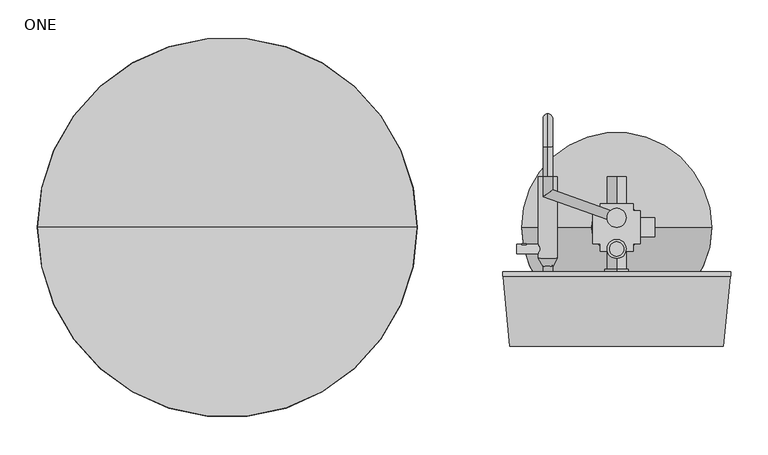
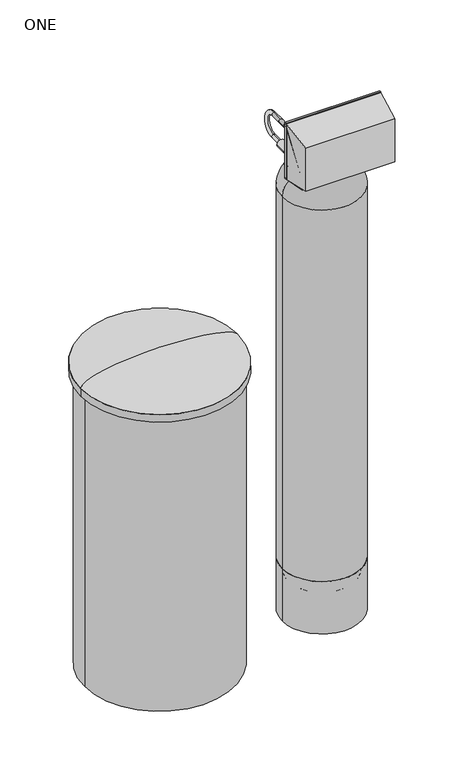
"""IFC4 building model written with IfcOpenShell, lengths in millimetres: proxy geometry, Water_Softener-Single-Robert_B_Hill-Fiberglass : ONE."""

from ifc_helpers import new_model, si_unit, point, frame, frame_2d, origin, origin_with_axes, place, context, project, spatial, polyline, circle_curve, ellipse_curve, trimmed, segment, composite_curve, outline, extrude, faceted_brep, source, transform, mapped, element, save
from ifc_brep_helpers import plane_surface, cylinder_surface, revolved_surface, advanced_brep


def one_3beddf22(model_context):
    return source(origin(), model_context, "Body", "SolidModel", [
        extrude(outline(composite_curve([segment(trimmed(circle_curve(frame_2d((203.2, -28.956)), 9.525), [point((212.725, -28.956))], [point((193.675, -28.956))], False, "CARTESIAN"), True, "CONTINUOUS"), segment(trimmed(circle_curve(frame_2d((203.2, -28.956)), 9.525), [point((193.675, -28.956))], [point((212.725, -28.956))], False, "CARTESIAN"), True, "CONTINUOUS")], self_intersect=False)), frame((0.0, 0.0, 1608.455), z_axis=(0.0, 0.0, 1.0), x_axis=(1.0, 0.0, 0.0)), (0.0, 0.0, 1.0), 19.05),
        extrude(outline(composite_curve([segment(trimmed(circle_curve(frame_2d((0.0, 1581.15)), 9.525), [point((0.0, 1571.625))], [point((0.0, 1590.675))], False, "CARTESIAN"), True, "CONTINUOUS"), segment(trimmed(circle_curve(frame_2d((0.0, 1581.15)), 9.525), [point((0.0, 1590.675))], [point((0.0, 1571.625))], False, "CARTESIAN"), True, "CONTINUOUS")], self_intersect=False)), frame((231.775, 0.0, 0.0), z_axis=(1.0, 0.0, 0.0), x_axis=(0.0, 1.0, 0.0)), (0.0, 0.0, 1.0), 19.05),
        advanced_brep(
        [(203.2, -55.9279754, 1581.15), (203.2, -55.9279754, 1555.75), (203.2, -55.9279754, 1552.575), (203.2, -55.9279754, 1584.325), (203.2, 67.8970246, 1581.15), (203.2, 67.8970246, 1555.75), (203.2, 67.8970246, 1568.45), (203.2, -59.1029754, 1584.325), (203.2, -59.1029754, 1552.575), (203.2, -59.1029754, 1568.45)],
        [
            (0, 1, circle_curve(frame((203.2, -55.9279754, 1568.45), z_axis=(0.0, -1.0, 0.0), x_axis=(0.0, 0.0, -1.0)), 12.7)),
            (1, 2),
            (2, 3, circle_curve(frame((203.2, -55.9279754, 1568.45), z_axis=(0.0, 1.0, 0.0), x_axis=(0.0, 0.0, -1.0)), 15.875)),
            (3, 0),
            (1, 0, circle_curve(frame((203.2, -55.9279754, 1568.45), z_axis=(0.0, -1.0, 0.0), x_axis=(0.0, 0.0, -1.0)), 12.7)),
            (3, 2, circle_curve(frame((203.2, -55.9279754, 1568.45), z_axis=(0.0, 1.0, 0.0), x_axis=(0.0, 0.0, -1.0)), 15.875)),
            (4, 5, circle_curve(frame((203.2, 67.8970246, 1568.45), z_axis=(0.0, -1.0, 0.0), x_axis=(0.0, 0.0, -1.0)), 12.7)),
            (5, 1),
            (0, 4),
            (5, 4, circle_curve(frame((203.2, 67.8970246, 1568.45), z_axis=(0.0, -1.0, 0.0), x_axis=(0.0, 0.0, -1.0)), 12.7)),
            (6, 5),
            (4, 6),
            (7, 8, circle_curve(frame((203.2, -59.1029754, 1568.45), z_axis=(0.0, -1.0, 0.0), x_axis=(0.0, 0.0, -1.0)), 15.875)),
            (8, 9),
            (9, 7),
            (8, 7, circle_curve(frame((203.2, -59.1029754, 1568.45), z_axis=(0.0, -1.0, 0.0), x_axis=(0.0, 0.0, -1.0)), 15.875)),
            (2, 8),
            (7, 3),
        ],
        [
            plane_surface(frame((203.2, -55.9279754, 1568.45), z_axis=(0.0, 1.0, 0.0), x_axis=(0.0, 0.0, -1.0))),
            cylinder_surface(frame((203.2, -59.1029754, 1568.45), z_axis=(0.0, 1.0, 0.0), x_axis=(0.0, 0.0, -1.0)), 12.7),
            plane_surface(frame((203.2, 67.8970246, 1568.45), z_axis=(0.0, 1.0, 0.0), x_axis=(0.0, 0.0, -1.0))),
            plane_surface(frame((203.2, -59.1029754, 1568.45), z_axis=(0.0, -1.0, 0.0), x_axis=(0.0, 0.0, -1.0))),
            cylinder_surface(frame((203.2, -59.1029754, 1568.45), z_axis=(0.0, 1.0, 0.0), x_axis=(0.0, 0.0, -1.0)), 15.875),
        ],
        [
            (0, [[1, 2, 3, 4]]),
            (0, [[5, -4, 6, -2]]),
            (1, [[7, 8, -1, 9]]),
            (1, [[10, -9, -5, -8]]),
            (2, [[11, -7, 12]]),
            (2, [[-12, -10, -11]]),
            (3, [[13, 14, 15]]),
            (3, [[16, -15, -14]]),
            (4, [[-3, 17, -13, 18]]),
            (4, [[-6, -18, -16, -17]]),
        ],
    ),
        extrude(outline(polyline([(1738.3125, 355.6), (1738.3125, 50.8), (1552.575, 50.8), (1552.575, 355.6), (1738.3125, 355.6)]), holes=[polyline([(1558.925, 349.25), (1558.925, 57.15), (1731.9625, 57.15), (1731.9625, 349.25), (1558.925, 349.25)])]), frame((0.0, -65.4529754, 0.0), z_axis=(0.0, 1.0, 0.0), x_axis=(0.0, 0.0, 1.0)), (0.0, 0.0, 1.0), 6.35),
        faceted_brep([(346.075, -140.1006819, 1552.575), (346.075, -140.1006819, 1589.4295859), (60.325, -140.1006819, 1589.4295859), (60.325, -140.1006819, 1552.575), (355.6, -59.1029754, 1547.8125), (50.8, -59.1029754, 1547.8125), (50.8, -59.1029754, 1738.3125), (355.6, -59.1029754, 1738.3125)], [[[0, 1, 2, 3]], [[4, 5, 6, 7]], [[4, 7, 1, 0]], [[7, 6, 2, 1]], [[6, 5, 3, 2]], [[5, 4, 0, 3]]]),
        extrude(outline(composite_curve([segment(trimmed(circle_curve(frame_2d((203.2, 0.0)), 31.75), [point((171.45, 0.0))], [point((234.95, 0.0))], False, "CARTESIAN"), True, "CONTINUOUS"), segment(trimmed(circle_curve(frame_2d((203.2, 0.0)), 31.75), [point((234.95, 0.0))], [point((171.45, 0.0))], False, "CARTESIAN"), True, "CONTINUOUS")], self_intersect=False)), frame((0.0, 0.0, 1536.7), z_axis=(0.0, 0.0, 1.0), x_axis=(1.0, 0.0, 0.0)), (0.0, 0.0, 1.0), 24.1545859),
        faceted_brep([(60.325, -159.1154754, 1706.9045859), (60.325, -159.1154754, 1560.8545859), (346.075, -159.1154754, 1560.8545859), (346.075, -159.1154754, 1706.9045859), (50.8, -59.1029754, 1738.3125), (355.6, -59.1029754, 1738.3125), (355.6, -59.1029754, 1547.8125), (50.8, -59.1029754, 1547.8125)], [[[0, 1, 2, 3]], [[4, 5, 6, 7]], [[4, 7, 1, 0]], [[7, 6, 2, 1]], [[6, 5, 3, 2]], [[5, 4, 0, 3]]]),
        extrude(outline(composite_curve([segment(trimmed(circle_curve(frame_2d((1568.45, 111.125)), 6.35), [point((1568.45, 117.475))], [point((1568.45, 104.775))], False, "CARTESIAN"), True, "CONTINUOUS"), segment(trimmed(circle_curve(frame_2d((1568.45, 111.125)), 6.35), [point((1568.45, 104.775))], [point((1568.45, 117.475))], False, "CARTESIAN"), True, "CONTINUOUS")], self_intersect=False)), frame((0.0, -59.1029754, 0.0), z_axis=(0.0, 1.0, 0.0), x_axis=(0.0, 0.0, 1.0)), (0.0, 0.0, 1.0), 17.4625),
        extrude(outline(composite_curve([segment(trimmed(circle_curve(frame_2d((-28.9404754, 1568.45)), 6.35), [point((-35.2904754, 1568.45))], [point((-22.5904754, 1568.45))], False, "CARTESIAN"), True, "CONTINUOUS"), segment(trimmed(circle_curve(frame_2d((-28.9404754, 1568.45)), 6.35), [point((-22.5904754, 1568.45))], [point((-35.2904754, 1568.45))], False, "CARTESIAN"), True, "CONTINUOUS")], self_intersect=False)), frame((69.85, 0.0, 0.0), z_axis=(1.0, 0.0, 0.0), x_axis=(0.0, 1.0, 0.0)), (0.0, 0.0, 1.0), 41.275),
        extrude(outline(composite_curve([segment(trimmed(circle_curve(frame_2d((1568.45, 111.125)), 12.7), [point((1568.45, 98.425))], [point((1568.45, 123.825))], False, "CARTESIAN"), True, "CONTINUOUS"), segment(trimmed(circle_curve(frame_2d((1568.45, 111.125)), 12.7), [point((1568.45, 123.825))], [point((1568.45, 98.425))], False, "CARTESIAN"), True, "CONTINUOUS")], self_intersect=False)), frame((0.0, -41.6404754, 0.0), z_axis=(0.0, 1.0, 0.0), x_axis=(0.0, 0.0, 1.0)), (0.0, 0.0, 1.0), 109.5375),
        advanced_brep(
        [(98.425, -41.6404754, 1568.45), (123.825, -41.6404754, 1568.45), (104.775, -52.7529754, 1568.45), (117.475, -52.7529754, 1568.45)],
        [
            (0, 1, circle_curve(frame((111.125, -41.6404754, 1568.45), z_axis=(0.0, 1.0, 0.0), x_axis=(-1.0, 0.0, 0.0)), 12.7)),
            (1, 0, circle_curve(frame((111.125, -41.6404754, 1568.45), z_axis=(0.0, 1.0, 0.0), x_axis=(1.0, 0.0, 0.0)), 12.7)),
            (2, 3, circle_curve(frame((111.125, -52.7529754, 1568.45), z_axis=(0.0, -1.0, 0.0), x_axis=(1.0, 0.0, 0.0)), 6.35)),
            (3, 2, circle_curve(frame((111.125, -52.7529754, 1568.45), z_axis=(0.0, -1.0, 0.0), x_axis=(-1.0, 0.0, 0.0)), 6.35)),
            (2, 0),
            (1, 3),
        ],
        [
            plane_surface(frame((111.125, -41.6404754, 1568.45), z_axis=(0.0, 1.0, 0.0), x_axis=(0.0, 0.0, -1.0))),
            plane_surface(frame((111.125, -52.7529754, 1568.45), z_axis=(0.0, -1.0, 0.0), x_axis=(0.0, 0.0, -1.0))),
            revolved_surface(polyline([(104.77499999999999, -52.7529754, 1568.45), (98.425, -41.6404754, 1568.45)]), (111.125, -63.8654754, 1568.45), (0.0, 1.0, 0.0)),
            revolved_surface(polyline([(117.47500000000001, -52.7529754, 1568.45), (123.825, -41.6404754, 1568.45)]), (111.125, -63.8654754, 1568.45), (0.0, 1.0, 0.0)),
        ],
        [
            (0, [[1, 2]]),
            (1, [[3, 4]]),
            (2, [[-3, 5, -2, 6]]),
            (3, [[-4, -6, -1, -5]]),
        ],
    ),
        extrude(outline(composite_curve([segment(trimmed(circle_curve(frame_2d((203.2, 12.7)), 12.7), [point((190.5, 12.7))], [point((215.9, 12.7))], False, "CARTESIAN"), True, "CONTINUOUS"), segment(trimmed(circle_curve(frame_2d((203.2, 12.7)), 12.7), [point((215.9, 12.7))], [point((190.5, 12.7))], False, "CARTESIAN"), True, "CONTINUOUS")], self_intersect=False)), frame((0.0, 0.0, 1600.2), z_axis=(0.0, 0.0, 1.0), x_axis=(1.0, 0.0, 0.0)), (0.0, 0.0, 1.0), 60.325),
        advanced_brep(
        [(104.775, 67.8970246, 1644.65), (117.475, 67.8970246, 1644.65), (104.775, 41.2010874, 1644.65), (117.475, 50.1429618, 1644.65), (201.0591918, 6.7217527, 1644.65), (205.3408082, 18.6782473, 1644.65)],
        [
            (0, 1, circle_curve(frame((111.125, 67.8970246, 1644.65), z_axis=(0.0, 1.0, 0.0), x_axis=(1.0, 0.0, 0.0)), 6.35)),
            (1, 0, circle_curve(frame((111.125, 67.8970246, 1644.65), z_axis=(0.0, 1.0, 0.0), x_axis=(1.0, 0.0, 0.0)), 6.35)),
            (0, 2),
            (2, 3, ellipse_curve(frame((111.125, 45.6720246, 1644.65), z_axis=(-0.5757016803912287, 0.8176598163018136, 0.0), x_axis=(0.8176598163018136, 0.5757016803912287, 0.0)), 7.7660659, 6.35)),
            (3, 1),
            (3, 2, ellipse_curve(frame((111.125, 45.6720246, 1644.65), z_axis=(-0.5757016803912287, 0.8176598163018136, 0.0), x_axis=(0.8176598163018136, 0.5757016803912287, 0.0)), 7.7660659, 6.35)),
            (4, 5, circle_curve(frame((203.2, 12.7, 1644.65), z_axis=(0.941456260466675, -0.3371351503894311, 0.0), x_axis=(0.3371351503894311, 0.941456260466675, 0.0)), 6.35)),
            (5, 4, circle_curve(frame((203.2, 12.7, 1644.65), z_axis=(0.941456260466675, -0.3371351503894311, 0.0), x_axis=(0.3371351503894311, 0.941456260466675, 0.0)), 6.35)),
            (2, 4),
            (5, 3),
        ],
        [
            plane_surface(frame((111.125, 67.8970246, 1536.7), z_axis=(0.0, 1.0, 0.0), x_axis=(0.0, 0.0, 1.0))),
            cylinder_surface(frame((111.125, 67.8970246, 1644.65), z_axis=(0.0, 1.0, 0.0), x_axis=(1.0, 0.0, 0.0)), 6.35),
            plane_surface(frame((203.2, 12.7, 1536.7), z_axis=(0.941456260466675, -0.3371351503894311, 0.0), x_axis=(0.0, 0.0, 1.0))),
            cylinder_surface(frame((111.125, 45.6720246, 1644.65), z_axis=(-0.941456260466675, 0.3371351503894311, 0.0), x_axis=(0.3371351503894311, 0.941456260466675, 0.0)), 6.35),
        ],
        [
            (0, [[1, 2]]),
            (1, [[-1, 3, 4, 5]]),
            (1, [[-2, -5, 6, -3]]),
            (2, [[7, 8]]),
            (3, [[-4, 9, -8, 10]]),
            (3, [[-6, -10, -7, -9]]),
        ],
    ),
        advanced_brep(
        [(111.125, -59.1029754, 1562.1), (111.125, -59.1029754, 1574.8), (111.125, 107.5845246, 1562.1), (111.125, 107.5845246, 1574.8), (111.125, 107.5845246, 1638.3), (111.125, 107.5845246, 1651.0), (111.125, 67.8970246, 1651.0), (111.125, 67.8970246, 1638.3)],
        [
            (0, 1, circle_curve(frame((111.125, -59.1029754, 1568.45), z_axis=(0.0, -1.0, 0.0), x_axis=(0.0, 0.0, 1.0)), 6.35)),
            (1, 0, circle_curve(frame((111.125, -59.1029754, 1568.45), z_axis=(0.0, -1.0, 0.0), x_axis=(0.0, 0.0, 1.0)), 6.35)),
            (0, 2),
            (2, 3, circle_curve(frame((111.125, 107.5845246, 1568.45), z_axis=(0.0, -1.0, 0.0), x_axis=(0.0, 0.0, 1.0)), 6.35)),
            (3, 1),
            (3, 2, circle_curve(frame((111.125, 107.5845246, 1568.45), z_axis=(0.0, -1.0, 0.0), x_axis=(0.0, 0.0, 1.0)), 6.35)),
            (4, 3, circle_curve(frame((111.125, 107.5845246, 1606.55), z_axis=(-1.0, 0.0, 0.0), x_axis=(0.0, 0.0, -1.0)), 31.75)),
            (2, 5, circle_curve(frame((111.125, 107.5845246, 1606.55), z_axis=(1.0, 0.0, 0.0), x_axis=(0.0, 0.0, -1.0)), 44.45)),
            (5, 4, circle_curve(frame((111.125, 107.5845246, 1644.65), z_axis=(0.0, 1.0, 0.0), x_axis=(0.0, 0.0, -1.0)), 6.35)),
            (4, 5, circle_curve(frame((111.125, 107.5845246, 1644.65), z_axis=(0.0, 1.0, 0.0), x_axis=(0.0, 0.0, -1.0)), 6.35)),
            (6, 7, circle_curve(frame((111.125, 67.8970246, 1644.65), z_axis=(0.0, -1.0, 0.0), x_axis=(0.0, 0.0, -1.0)), 6.35)),
            (7, 6, circle_curve(frame((111.125, 67.8970246, 1644.65), z_axis=(0.0, -1.0, 0.0), x_axis=(0.0, 0.0, -1.0)), 6.35)),
            (5, 6),
            (7, 4),
        ],
        [
            plane_surface(frame((203.2, -59.1029754, 1568.45), z_axis=(0.0, -1.0, 0.0), x_axis=(1.0, 0.0, 0.0))),
            cylinder_surface(frame((111.125, -59.1029754, 1568.45), z_axis=(0.0, -1.0, 0.0), x_axis=(0.0, 0.0, 1.0)), 6.35),
            revolved_surface(trimmed(ellipse_curve(frame((111.125, 107.5845246, 1568.45), z_axis=(0.0, -1.0, 0.0), x_axis=(0.0, 0.0, 1.0)), 6.35, 6.35), [point((111.125, 107.5845246, 1562.1))], [point((111.125, 107.5845246, 1574.8))], True, "CARTESIAN"), (203.2, 107.5845246, 1606.55), (1.0, 0.0, 0.0)),
            revolved_surface(trimmed(ellipse_curve(frame((111.125, 107.5845246, 1568.45), z_axis=(0.0, -1.0, 0.0), x_axis=(0.0, 0.0, 1.0)), 6.35, 6.35), [point((111.125, 107.5845246, 1574.8))], [point((111.125, 107.5845246, 1562.1))], True, "CARTESIAN"), (203.2, 107.5845246, 1606.55), (1.0, 0.0, 0.0)),
            plane_surface(frame((203.2, 67.8970246, 1644.65), z_axis=(0.0, -1.0, 0.0), x_axis=(1.0, 0.0, 0.0))),
            cylinder_surface(frame((111.125, 107.5845246, 1644.65), z_axis=(0.0, 1.0, 0.0), x_axis=(0.0, 0.0, -1.0)), 6.35),
        ],
        [
            (0, [[1, 2]]),
            (1, [[-1, 3, 4, 5]]),
            (1, [[-2, -5, 6, -3]]),
            (2, [[7, -4, 8, 9]]),
            (3, [[-8, -6, -7, 10]]),
            (4, [[11, 12]]),
            (5, [[-9, 13, -12, 14]]),
            (5, [[-10, -14, -11, -13]]),
        ],
    ),
        extrude(outline(polyline([(180.975, 22.225), (180.975, 31.75), (225.425, 31.75), (225.425, 22.225), (234.95, 22.225), (234.95, -22.225), (225.425, -22.225), (225.425, -31.75), (180.975, -31.75), (180.975, -22.225), (171.45, -22.225), (171.45, 22.225), (180.975, 22.225)])), frame((0.0, 0.0, 1552.575), z_axis=(0.0, 0.0, 1.0), x_axis=(1.0, 0.0, 0.0)), (0.0, 0.0, 1.0), 47.625),
        extrude(outline(composite_curve([segment(trimmed(circle_curve(frame_2d((203.2, -28.9404754)), 12.7), [point((190.5, -28.9404754))], [point((215.9, -28.9404754))], False, "CARTESIAN"), True, "CONTINUOUS"), segment(trimmed(circle_curve(frame_2d((203.2, -28.9404754)), 12.7), [point((215.9, -28.9404754))], [point((190.5, -28.9404754))], False, "CARTESIAN"), True, "CONTINUOUS")], self_intersect=False)), frame((0.0, 0.0, 1568.45), z_axis=(0.0, 0.0, 1.0), x_axis=(1.0, 0.0, 0.0)), (0.0, 0.0, 1.0), 59.0795859),
        extrude(outline(composite_curve([segment(trimmed(circle_curve(frame_2d((0.0, 1581.15)), 12.7), [point((-12.7, 1581.15))], [point((12.7, 1581.15))], False, "CARTESIAN"), True, "CONTINUOUS"), segment(trimmed(circle_curve(frame_2d((0.0, 1581.15)), 12.7), [point((12.7, 1581.15))], [point((-12.7, 1581.15))], False, "CARTESIAN"), True, "CONTINUOUS")], self_intersect=False)), frame((234.95, 0.0, 0.0), z_axis=(1.0, 0.0, 0.0), x_axis=(0.0, 1.0, 0.0)), (0.0, 0.0, 1.0), 19.05),
        advanced_brep(
        [(76.2, 0.0, 0.0), (330.2, 0.0, 0.0), (311.15, 0.0, 0.0), (95.25, 0.0, 0.0), (76.2, 0.0, 177.8), (330.2, 0.0, 177.8), (95.25, 0.0, 177.8), (311.15, 0.0, 177.8)],
        [
            (0, 1, circle_curve(frame((203.2, 0.0, 0.0), z_axis=(0.0, 0.0, -1.0), x_axis=(1.0, 0.0, 0.0)), 127.0)),
            (1, 2),
            (2, 3, circle_curve(frame((203.2, 0.0, 0.0), z_axis=(0.0, 0.0, 1.0), x_axis=(1.0, 0.0, 0.0)), 107.95)),
            (3, 0),
            (1, 0, circle_curve(frame((203.2, 0.0, 0.0), z_axis=(0.0, 0.0, -1.0), x_axis=(1.0, 0.0, 0.0)), 127.0)),
            (3, 2, circle_curve(frame((203.2, 0.0, 0.0), z_axis=(0.0, 0.0, 1.0), x_axis=(1.0, 0.0, 0.0)), 107.95)),
            (4, 5, circle_curve(frame((203.2, 0.0, 177.8), z_axis=(0.0, 0.0, -1.0), x_axis=(1.0, 0.0, 0.0)), 127.0)),
            (5, 1),
            (0, 4),
            (5, 4, circle_curve(frame((203.2, 0.0, 177.8), z_axis=(0.0, 0.0, -1.0), x_axis=(1.0, 0.0, 0.0)), 127.0)),
            (6, 7, circle_curve(frame((203.2, 0.0, 177.8), z_axis=(0.0, 0.0, -1.0), x_axis=(1.0, 0.0, 0.0)), 107.95)),
            (7, 5),
            (4, 6),
            (7, 6, circle_curve(frame((203.2, 0.0, 177.8), z_axis=(0.0, 0.0, -1.0), x_axis=(1.0, 0.0, 0.0)), 107.95)),
            (2, 7),
            (6, 3),
        ],
        [
            plane_surface(frame((203.2, 0.0, 0.0), z_axis=(0.0, 0.0, -1.0), x_axis=(1.0, 0.0, 0.0))),
            cylinder_surface(frame((203.2, 0.0, 177.8), z_axis=(0.0, 0.0, 1.0), x_axis=(1.0, 0.0, 0.0)), 127.0),
            plane_surface(frame((203.2, 0.0, 177.8), z_axis=(0.0, 0.0, 1.0), x_axis=(1.0, 0.0, 0.0))),
            revolved_surface(polyline([(311.15, 0.0, 177.8), (311.15, 0.0, 0.0)]), (203.2, 0.0, 177.8), (0.0, 0.0, 1.0)),
        ],
        [
            (0, [[1, 2, 3, 4]]),
            (0, [[5, -4, 6, -2]]),
            (1, [[7, 8, -1, 9]]),
            (1, [[10, -9, -5, -8]]),
            (2, [[11, 12, -7, 13]]),
            (2, [[14, -13, -10, -12]]),
            (3, [[-3, 15, -11, 16]]),
            (3, [[-6, -16, -14, -15]]),
        ],
    ),
        advanced_brep(
        [(203.2, 0.0, 1549.4), (236.5375, 0.0, 1549.4), (169.8625, 0.0, 1549.4), (161.925, 0.0, 59.4375), (244.475, 0.0, 59.4375), (203.2, 0.0, 59.4375), (161.925, 0.0, 89.8788701), (244.475, 0.0, 89.8788701), (76.2, 0.0, 177.8), (330.2, 0.0, 177.8), (76.2, 0.0, 1439.76875), (330.2, 0.0, 1439.76875), (169.8625, 0.0, 1526.0463622), (236.5375, 0.0, 1526.0463622)],
        [
            (0, 1),
            (1, 2, circle_curve(frame((203.2, 0.0, 1549.4), z_axis=(0.0, 0.0, 1.0), x_axis=(1.0, 0.0, 0.0)), 33.3375)),
            (2, 0),
            (2, 1, circle_curve(frame((203.2, 0.0, 1549.4), z_axis=(0.0, 0.0, 1.0), x_axis=(1.0, 0.0, 0.0)), 33.3375)),
            (3, 4, circle_curve(frame((203.2, 0.0, 59.4375), z_axis=(0.0, 0.0, -1.0), x_axis=(1.0, 0.0, 0.0)), 41.275)),
            (4, 5),
            (5, 3),
            (4, 3, circle_curve(frame((203.2, 0.0, 59.4375), z_axis=(0.0, 0.0, -1.0), x_axis=(1.0, 0.0, 0.0)), 41.275)),
            (6, 7, circle_curve(frame((203.2, 0.0, 89.8788701), z_axis=(0.0, 0.0, -1.0), x_axis=(1.0, 0.0, 0.0)), 41.275)),
            (7, 4),
            (3, 6),
            (7, 6, circle_curve(frame((203.2, 0.0, 89.8788701), z_axis=(0.0, 0.0, -1.0), x_axis=(1.0, 0.0, 0.0)), 41.275)),
            (8, 9, circle_curve(frame((203.2, 0.0, 177.8), z_axis=(0.0, 0.0, -1.0), x_axis=(1.0, 0.0, 0.0)), 127.0)),
            (9, 7, ellipse_curve(frame((203.2, 0.0, 177.8), z_axis=(0.0, 1.0, 0.0), x_axis=(-1.0, 0.0, 0.0)), 127.0, 92.9679887)),
            (6, 8, ellipse_curve(frame((203.2, 0.0, 177.8), z_axis=(0.0, 1.0, 0.0), x_axis=(1.0, 0.0, 0.0)), 127.0, 92.9679887)),
            (9, 8, circle_curve(frame((203.2, 0.0, 177.8), z_axis=(0.0, 0.0, -1.0), x_axis=(1.0, 0.0, 0.0)), 127.0)),
            (10, 11, circle_curve(frame((203.2, 0.0, 1439.76875), z_axis=(0.0, 0.0, -1.0), x_axis=(1.0, 0.0, 0.0)), 127.0)),
            (11, 9),
            (8, 10),
            (11, 10, circle_curve(frame((203.2, 0.0, 1439.76875), z_axis=(0.0, 0.0, -1.0), x_axis=(1.0, 0.0, 0.0)), 127.0)),
            (12, 13, circle_curve(frame((203.2, 0.0, 1526.0463622), z_axis=(0.0, 0.0, -1.0), x_axis=(1.0, 0.0, 0.0)), 33.3375)),
            (13, 11, ellipse_curve(frame((203.2, 0.0, 1439.76875), z_axis=(0.0, 1.0, 0.0), x_axis=(1.0, 0.0, 0.0)), 127.0, 89.4131533)),
            (10, 12, ellipse_curve(frame((203.2, 0.0, 1439.76875), z_axis=(0.0, 1.0, 0.0), x_axis=(-1.0, 0.0, 0.0)), 127.0, 89.4131533)),
            (13, 12, circle_curve(frame((203.2, 0.0, 1526.0463622), z_axis=(0.0, 0.0, -1.0), x_axis=(1.0, 0.0, 0.0)), 33.3375)),
            (1, 13),
            (12, 2),
        ],
        [
            plane_surface(frame((203.2, 0.0, 1549.4), z_axis=(0.0, 0.0, 1.0), x_axis=(1.0, 0.0, 0.0))),
            plane_surface(frame((203.2, 0.0, 59.4375), z_axis=(0.0, 0.0, -1.0), x_axis=(1.0, 0.0, 0.0))),
            cylinder_surface(frame((203.2, 0.0, 2486.3581012), z_axis=(0.0, 0.0, 1.0), x_axis=(1.0, 0.0, 0.0)), 41.275),
            revolved_surface(trimmed(ellipse_curve(frame((203.2, 0.0, 177.8), z_axis=(0.0, -1.0, 0.0), x_axis=(0.0, 0.0, 1.0)), 92.9679887, 127.0), [point((244.475, 0.0, 89.8788701))], [point((330.2, 0.0, 177.8))], True, "CARTESIAN"), (203.2, 0.0, 2486.3581012), (0.0, 0.0, 1.0)),
            cylinder_surface(frame((203.2, 0.0, 2486.3581012), z_axis=(0.0, 0.0, 1.0), x_axis=(1.0, 0.0, 0.0)), 127.0),
            revolved_surface(trimmed(ellipse_curve(frame((203.2, 0.0, 1439.76875), z_axis=(0.0, -1.0, 0.0), x_axis=(0.0, 0.0, -1.0)), 89.4131533, 127.0), [point((330.2, 0.0, 1439.76875))], [point((236.5375, 0.0, 1526.0463622))], True, "CARTESIAN"), (203.2, 0.0, 2486.3581012), (0.0, 0.0, 1.0)),
            cylinder_surface(frame((203.2, 0.0, 2486.3581012), z_axis=(0.0, 0.0, 1.0), x_axis=(1.0, 0.0, 0.0)), 33.3375),
        ],
        [
            (0, [[1, 2, 3]]),
            (0, [[-3, 4, -1]]),
            (1, [[5, 6, 7]]),
            (1, [[8, -7, -6]]),
            (2, [[9, 10, -5, 11]]),
            (2, [[12, -11, -8, -10]]),
            (3, [[13, 14, -9, 15]]),
            (3, [[16, -15, -12, -14]]),
            (4, [[17, 18, -13, 19]]),
            (4, [[20, -19, -16, -18]]),
            (5, [[21, 22, -17, 23]]),
            (5, [[24, -23, -20, -22]]),
            (6, [[-2, 25, -21, 26]]),
            (6, [[-4, -26, -24, -25]]),
        ],
    ),
        extrude(outline(composite_curve([segment(trimmed(circle_curve(frame_2d((-317.5, 0.0)), 254.0), [point((-63.5, 0.0))], [point((-571.5, 0.0))], False, "CARTESIAN"), True, "CONTINUOUS"), segment(trimmed(circle_curve(frame_2d((-317.5, 0.0)), 254.0), [point((-571.5, 0.0))], [point((-63.5, 0.0))], False, "CARTESIAN"), True, "CONTINUOUS")], self_intersect=False)), frame((0.0, 0.0, 990.6), z_axis=(0.0, 0.0, 1.0), x_axis=(1.0, 0.0, 0.0)), (0.0, 0.0, 1.0), 25.4),
        advanced_brep(
        [(-571.5, 0.0, 1016.0), (-63.5, 0.0, 1016.0), (-317.5, 0.0, 1066.8), (-317.5, 0.0, 1016.0)],
        [
            (0, 1, circle_curve(frame((-317.5, 0.0, 1016.0), z_axis=(0.0, 0.0, 1.0), x_axis=(1.0, 0.0, 0.0)), 254.0)),
            (1, 2, ellipse_curve(frame((-317.5, 0.0, 1016.0), z_axis=(0.0, -1.0, 0.0), x_axis=(1.0, 0.0, 0.0)), 254.0, 50.8)),
            (2, 0, ellipse_curve(frame((-317.5, 0.0, 1016.0), z_axis=(0.0, -1.0, 0.0), x_axis=(-1.0, 0.0, 0.0)), 254.0, 50.8)),
            (1, 0, circle_curve(frame((-317.5, 0.0, 1016.0), z_axis=(0.0, 0.0, 1.0), x_axis=(1.0, 0.0, 0.0)), 254.0)),
            (3, 1),
            (0, 3),
        ],
        [
            revolved_surface(trimmed(ellipse_curve(frame((-317.5, 0.0, 1016.0), z_axis=(0.0, 0.9999999999999999, 0.0), x_axis=(1.0, 0.0, 0.0)), 254.0, 50.8), [point((-317.5, 0.0, 1066.8))], [point((-63.5, 0.0, 1016.0))], True, "CARTESIAN"), (-317.5, 0.0, 1066.8), (0.0, 0.0, -0.9999999999999999)),
            plane_surface(frame((-317.5, 0.0, 1016.0), z_axis=(0.0, 0.0, -1.0), x_axis=(1.0, 0.0, 0.0))),
        ],
        [
            (0, [[1, 2, 3]]),
            (0, [[4, -3, -2]]),
            (1, [[5, -1, 6]]),
            (1, [[-6, -4, -5]]),
        ],
    ),
        extrude(outline(composite_curve([segment(trimmed(circle_curve(frame_2d((-317.5, 0.0)), 241.3), [point((-76.2, 0.0))], [point((-558.8, 0.0))], False, "CARTESIAN"), True, "CONTINUOUS"), segment(trimmed(circle_curve(frame_2d((-317.5, 0.0)), 241.3), [point((-558.8, 0.0))], [point((-76.2, 0.0))], False, "CARTESIAN"), True, "CONTINUOUS")], self_intersect=False)), origin_with_axes(), (0.0, 0.0, 1.0), 990.6),
        extrude(outline(composite_curve([segment(trimmed(circle_curve(frame_2d((0.0, 939.8)), 12.7), [point((12.7, 939.8))], [point((-12.7, 939.8))], False, "CARTESIAN"), True, "CONTINUOUS"), segment(trimmed(circle_curve(frame_2d((0.0, 939.8)), 12.7), [point((-12.7, 939.8))], [point((12.7, 939.8))], False, "CARTESIAN"), True, "CONTINUOUS")], self_intersect=False)), frame((-82.55, 0.0, 0.0), z_axis=(1.0, 0.0, 0.0), x_axis=(0.0, 1.0, 0.0)), (0.0, 0.0, 1.0), 12.7),
        extrude(outline(composite_curve([segment(trimmed(circle_curve(frame_2d((0.0, 863.6)), 25.4), [point((25.4, 863.6))], [point((-25.4, 863.6))], False, "CARTESIAN"), True, "CONTINUOUS"), segment(trimmed(circle_curve(frame_2d((0.0, 863.6)), 25.4), [point((-25.4, 863.6))], [point((25.4, 863.6))], False, "CARTESIAN"), True, "CONTINUOUS")], self_intersect=False)), frame((-82.55, 0.0, 0.0), z_axis=(1.0, 0.0, 0.0), x_axis=(0.0, 1.0, 0.0)), (0.0, 0.0, 1.0), 12.7),
        extrude(outline(composite_curve([segment(trimmed(circle_curve(frame_2d((1568.45, 203.2)), 12.636392), [point((1568.45, 190.563608))], [point((1568.45, 215.836392))], False, "CARTESIAN"), True, "CONTINUOUS"), segment(trimmed(circle_curve(frame_2d((1568.45, 203.2)), 12.636392), [point((1568.45, 215.836392))], [point((1568.45, 190.563608))], False, "CARTESIAN"), True, "CONTINUOUS")], self_intersect=False)), frame((0.0, 60.325, 0.0), z_axis=(0.0, 1.0, 0.0), x_axis=(0.0, 0.0, 1.0)), (0.0, 0.0, 1.0), 6.35),
        extrude(outline(composite_curve([segment(trimmed(circle_curve(frame_2d((-28.575, 1568.45)), 6.35), [point((-34.925, 1568.45))], [point((-22.225, 1568.45))], False, "CARTESIAN"), True, "CONTINUOUS"), segment(trimmed(circle_curve(frame_2d((-28.575, 1568.45)), 6.35), [point((-22.225, 1568.45))], [point((-34.925, 1568.45))], False, "CARTESIAN"), True, "CONTINUOUS")], self_intersect=False)), frame((76.2, 0.0, 0.0), z_axis=(1.0, 0.0, 0.0), x_axis=(0.0, 1.0, 0.0)), (0.0, 0.0, 1.0), 6.35),
    ])


if __name__ == "__main__":
    model = new_model("IFC4")
    model_context = context("Model", 3, world=origin())
    ifc_project = project(units=[si_unit("LENGTHUNIT", "METRE", prefix="MILLI")], contexts=[model_context])
    site = spatial("IfcSite", under=ifc_project)
    building = spatial("IfcBuilding", under=site)
    placement = place(None, origin())
    one_shape = one_3beddf22(model_context)
    element("IfcBuildingElementProxy", 1, Name="Water_Softener-Single-Robert_B_Hill-Fiberglass : ONE", ObjectType="Water_Softener-Single-Robert_B_Hill-Fiberglass : ONE", at=placement, inside=building, context=model_context, shape_type="MappedRepresentation", body=[
        mapped(one_shape, transform((0.0, 0.0, 0.0), x_axis=(1.0, 0.0, 0.0), y_axis=(0.0, 1.0, 0.0), z_axis=(0.0, 0.0, 1.0))),
    ])
    save(model, "model.ifc")

# Revit data of these elements
# Type "Water_Softener-Single-Robert_B_Hill-Fiberglass : ONE"
#   URL = "www.hillwater.com"
#   Type Comments = "Single Fiberglass, 1in, 120VAC Electrical Service Required 6ft From Softener, 24\" Clearance Above Softener For Access"
#   Connector 5 Description = "Brine To Softener Out"
#   Product Page URL = ""
#   Product Documentation Link = ""
#   Model = "HICAP-0090-1"
#   Manufacturer = "Robert B. Hill Co."
#   Description = "Single Fiberglass"
#   Copyright © = "© Robert B. Hill Co."
#   Connector 14 Description = "Drainage"
#   Connector 7 Description = "Softener To Brine In"
#   Connector 15 Description = "Domestic Cold Water Outlet"
#   Connector 8 Description = "Domestic Cold Water Inlet"
#   Connector 16 Description = "Power"
#   Brine Tank Salt Storage = "400lbs."
#   Assembly Code = "D2090600"
#   Water Softener Radius = 0' - 5"
#   Softener Height = 4' - 6"
#   Softener Diameter = 0' - 10"
#   Voltage = 120 V
#   Valve Drain Radius = 0' - 0 1/2"
#   Upper Outlet left Right Connector Distance = 0' - 0"
#   Upper Outlet Radius = 0' - 0 1/2"
#   Upper Outlet Height From Tank = 0' - 0"
#   Upper Outlet Front Back Distance = 0' - 0"
#   Tank Opening Diameter = 0' - 2 5/8"
#   Tank Drain Radius = 0' - 0 1/2"
#   Resin Per Tank = 2 (stored number, unit not read)
#   Power Left Right Distance = 0' - 5"
#   Power Front Back Distance = 0' - 4 1/2"
#   Power From Tank Height = 0' - 2 1/2"
#   Outlet Angle = 90.00°
#   CTRL Brine Overflow Diameter = 0' - 1"
#   Pressure Drop [instance default] = 25.00 psi
#   Power Factor = 0
#   Overal Height = 5' - 1"
#   Outlet Height From Tank = 0' - 2.7"
#   Outlet Left Right Connector Distance = 0' - 0"
#   Outlet Front Back Distance = 0' - 1.14"
#   Inlet Outlet Radius = 0' - 0 1/2"
#   Inlet Front Back Distance = 0' - 2 5/8"
#   Inlet Connector Height From Tank = 0' - 0 3/4"
#   Flow [instance default] = 22 GPM
#   Drain Left Right Distance = 0' - 5"
#   Drain Height From tank = 0' - 1 1/4"
#   Drain Front Back Distance = 0' - 0"
#   Distance Apart = 0' - 6"
#   Connection Size = 0' - 1"
#   CTRL Drain Connector Angle = 0.00°
#   CTRL Distance Apart [instance default] = 0' - 6"
#   Brine Tank Radius = 0' - 9 1/2"
#   Brine Tank Height = 3' - 4"
#   Brine Tank Diameter = 1' - 7"
#   Brine Overflow Diameter = 0' - 1"
#   Brine Connector Radius = 0' - 0 1/4"
#   Brine Front Back Connector Distance = 0' - 1 1/8"
#   Brine Connector Height From Tank = 0' - 0 3/4"
#   Brine left Right Connector Distance = 0' - 5"
#   Base Height = 0' - 7"
#   Back Wash Flow Rate = 4 GPM
#   Apparent Load = 120 VA
#   25psi Drop = 22 GPM
#   15psi Drop = 18 GPM
#   Valve Type = 2750
#   Has 25psi Drop [instance default] = yes
#   Has 15psi Drop [instance default] = no
#   Number of Poles = 1
#   Has Tripod Base = no
#   Has Hybrid Base = no
#   Has Full Base = yes
#   Has 3900 Valve = no
#   Has 2900 Valve = no
#   Has 2850 Valve = no
#   Has 2750 Valve = yes
#   Base Type = 1
#   Softener Material [instance default] = Fiberglass - Robert B. Hill - Cream/Almond
#   Load Classification = Appliance - Dwelling Unit
#   Brine Tank Material = Polyethylene - Robert B. Hill - Black
# Element 1 (IfcBuildingElementProxy, "Water_Softener-Single-Robert_B_Hill-Fiberglass : ONE")
#   Materials on its faces: "Metal - Robert B. Hill - Brass", "Plastic - Robert B. Hill - Black", "Polyethylene - Robert B. Hill - Black", "Fiberglass - Robert B. Hill - Cream/Almond", "Metal - Robert B. Hill - Steel - Black"
# Materials
#   "Fiberglass - Robert B. Hill - Cream/Almond": class "Miscellaneous", colour RGB 255 255 179, transparency 0
#   "Polyethylene - Robert B. Hill - Black": class "Miscellaneous", colour RGB 0 0 0, transparency 0
#   "Metal - Robert B. Hill - Brass": class "Metal", colour RGB 202 154 58, transparency 0, Manufacturer = "Robert B. Hill", URL = "www.hillwater.com", Cost = 0
#   "Plastic - Robert B. Hill - Black": class "Plastic", colour RGB 5 5 5, transparency 0, Manufacturer = "Robert B. Hill", URL = "www.hillwater.com", Description = "Enviromental Cover", Cost = 0
#   "Metal - Robert B. Hill - Steel - Black": class "Plastic", colour RGB 5 5 5, transparency 0, Manufacturer = "Robert B. Hill", URL = "www.hillwater.com", Description = "Enviromental Cover", Cost = 0
